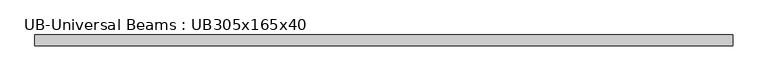
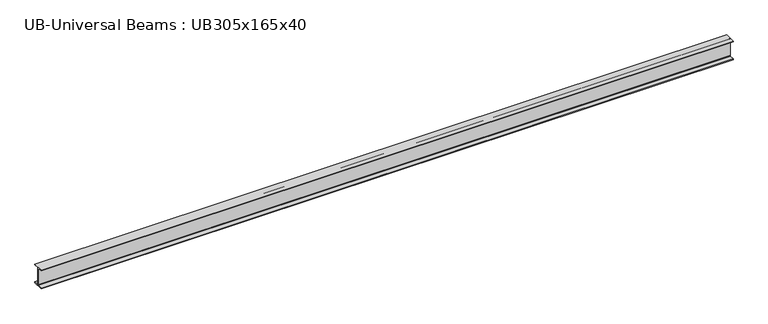
"""IFC4 building model written with IfcOpenShell, lengths in millimetres: beam geometry, UB-Universal Beams : UB305x165x40."""

from ifc_helpers import new_model, si_unit, point, frame, frame_2d, origin, place, context, project, spatial, polyline, circle_curve, trimmed, segment, composite_curve, outline, extrude, source, transform, mapped, element, save


def ub_universal_beams_ub305x165x40_321f4fc0(model_context):
    return source(origin(), model_context, "Body", "SweptSolid", [
        extrude(outline(composite_curve([segment(polyline([(82.5, -141.5), (82.5, -151.7), (-82.5, -151.7), (-82.5, -141.5), (-11.9, -141.5)]), True, "CONTINUOUS"), segment(trimmed(circle_curve(frame_2d((-11.9, -132.6)), 8.9), [point((-11.9, -141.5))], [point((-3.0, -132.6))], True, "CARTESIAN"), True, "CONTINUOUS"), segment(polyline([(-3.0, -132.6), (-3.0, 132.6)]), True, "CONTINUOUS"), segment(trimmed(circle_curve(frame_2d((-11.9, 132.6)), 8.9), [point((-3.0, 132.6))], [point((-11.9, 141.5))], True, "CARTESIAN"), True, "CONTINUOUS"), segment(polyline([(-11.9, 141.5), (-82.5, 141.5), (-82.5, 151.7), (82.5, 151.7), (82.5, 141.5), (11.9, 141.5)]), True, "CONTINUOUS"), segment(trimmed(circle_curve(frame_2d((11.9, 132.6)), 8.9), [point((11.9, 141.5))], [point((3.0, 132.6))], True, "CARTESIAN"), True, "CONTINUOUS"), segment(polyline([(3.0, 132.6), (3.0, -132.6)]), True, "CONTINUOUS"), segment(trimmed(circle_curve(frame_2d((11.9, -132.6)), 8.9), [point((3.0, -132.6))], [point((11.9, -141.5))], True, "CARTESIAN"), True, "CONTINUOUS"), segment(polyline([(11.9, -141.5), (82.5, -141.5)]), True, "CONTINUOUS")], self_intersect=False)), frame((-5147.55, 0.0, 0.0), z_axis=(1.0, 0.0, 0.0), x_axis=(0.0, 1.0, 0.0)), (0.0, 0.0, 1.0), 10718.6),
    ])


if __name__ == "__main__":
    model = new_model("IFC4")
    model_context = context("Model", 3, world=origin())
    ifc_project = project(units=[si_unit("LENGTHUNIT", "METRE", prefix="MILLI")], contexts=[model_context])
    site = spatial("IfcSite", under=ifc_project)
    building = spatial("IfcBuilding", under=site)
    placement = place(None, origin())
    ub_universal_beams_ub305x165x40_shape = ub_universal_beams_ub305x165x40_321f4fc0(model_context)
    element("IfcBeam", 1, ObjectType="UB-Universal Beams : UB305x165x40", at=placement, inside=building, context=model_context, shape_type="MappedRepresentation", body=[
        mapped(ub_universal_beams_ub305x165x40_shape, transform((0.0, 0.0, 0.0), x_axis=(1.0, 0.0, 0.0), y_axis=(0.0, 1.0, 0.0), z_axis=(0.0, 0.0, 1.0))),
    ])
    save(model, "model.ifc")

# Revit data of these elements
# Type "UB-Universal Beams : UB305x165x40"
#   Section Name Key = "UB305X165X40"
#   Width = 165 mm
#   Web Thickness = 6 mm
#   Web Fillet = 8.9 mm
#   Warping Constant = 164000 cm⁶
#   Torsional Moment of Inertia = 14.7 cm⁴
#   Section Area = 51.3 cm²
#   Plastic Modulus weak axis = 0.00501468 (stored number, unit not read)
#   Plastic Modulus strong axis = 0.022001 (stored number, unit not read)
#   Nominal Weight = 395.207 N/m
#   Moment of Inertia weak axis = 764 cm⁴
#   Moment of Inertia strong axis = 8503 cm⁴
#   Height = 303.4 mm
#   Flange Thickness = 10.2 mm
#   Elastic Modulus weak axis = 0.00327014 (stored number, unit not read)
#   Elastic Modulus strong axis = 0.0197762 (stored number, unit not read)
#   Centroid Vertical = 151.7 mm
#   Centroid Horizontal = 82.5 mm
#   Length [instance default] = 1500 mm
#   Structural Material [instance default] = Metal - Steel 43-275
#   Type Comments = ""
#   Assembly Code = ""
# Element 1 (IfcBeam, "UB-Universal Beams : UB305x165x40")
#   Materials on its faces: "Metal - Steel 43-275"
# Materials
#   "Metal - Steel 43-275": class "Metal", colour RGB 247 247 247, transparency 0, Cost = 0
